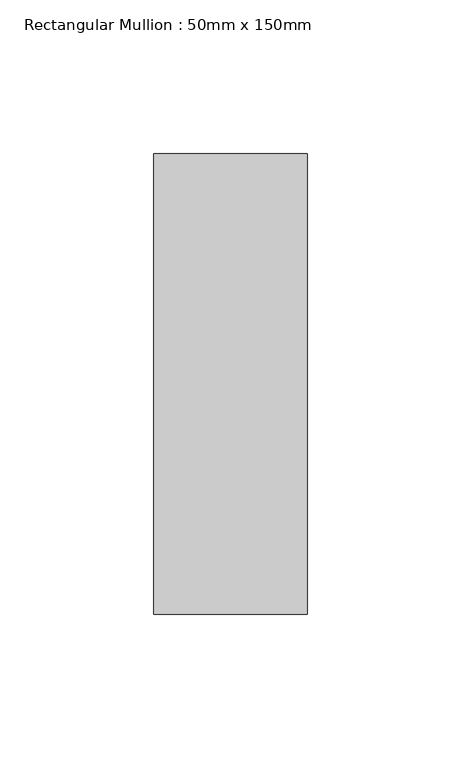
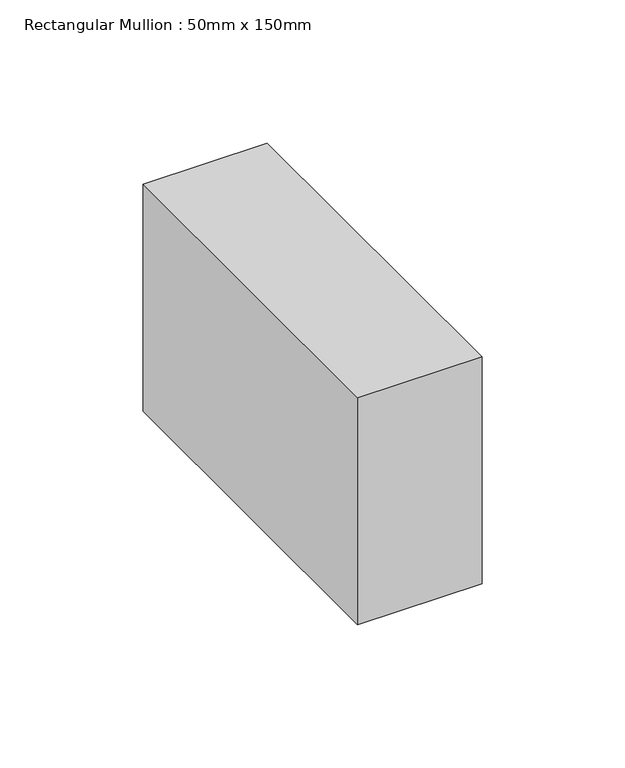
"""IFC4 building model written with IfcOpenShell, lengths in millimetres: member geometry, Rectangular Mullion : 50mm x 150mm."""

from ifc_helpers import new_model, si_unit, frame, origin, place, context, project, spatial, polyline, outline, extrude, source, transform, mapped, element, save


def rectangular_mullion_50mm_x_150mm_182d3367(model_context):
    return source(origin(), model_context, "Body", "SweptSolid", [
        extrude(outline(polyline([(25.0, 75.0), (25.0, -75.0), (-25.0, -75.0), (-25.0, 75.0), (25.0, 75.0)])), frame((0.0, 0.0, -96.8181816), z_axis=(0.0, 0.0, 1.0), x_axis=(1.0, 0.0, 0.0)), (0.0, 0.0, 1.0), 96.8181816),
    ])


if __name__ == "__main__":
    model = new_model("IFC4")
    model_context = context("Model", 3, world=origin())
    ifc_project = project(units=[si_unit("LENGTHUNIT", "METRE", prefix="MILLI")], contexts=[model_context])
    site = spatial("IfcSite", under=ifc_project)
    building = spatial("IfcBuilding", under=site)
    placement = place(None, origin())
    rectangular_mullion_50mm_x_150mm_shape = rectangular_mullion_50mm_x_150mm_182d3367(model_context)
    element("IfcMember", 1, ObjectType="Rectangular Mullion : 50mm x 150mm", at=placement, inside=building, context=model_context, shape_type="MappedRepresentation", body=[
        mapped(rectangular_mullion_50mm_x_150mm_shape, transform((0.0, 0.0, 0.0), x_axis=(1.0, 0.0, 0.0), y_axis=(0.0, 1.0, 0.0), z_axis=(0.0, 0.0, 1.0))),
    ])
    save(model, "model.ifc")

# Revit data of these elements
# Type "Rectangular Mullion : 50mm x 150mm"
#   built-in parameter 1007304 = 0.492126 (stored number, unit not read)
#   built-in parameter 1007301 = 0.082021 (stored number, unit not read)
#   built-in parameter 1007300 = 0.082021 (stored number, unit not read)
# Element 1 (IfcMember, "Rectangular Mullion : 50mm x 150mm")
#   Materials on its faces: "Aluminum"
# Materials
#   "Aluminum": class "Metal", colour RGB 244 244 244, transparency 0, Description = "Aluminum 6061", Cost = 0
